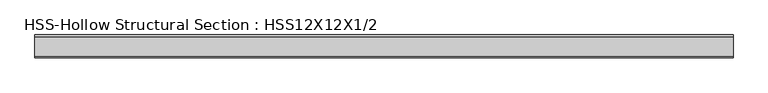
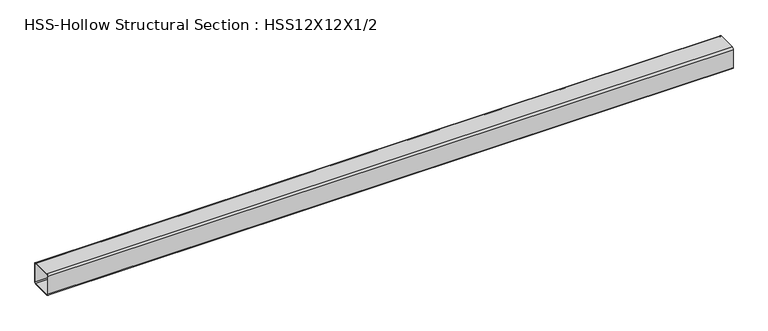
"""IFC4 building model written with IfcOpenShell, lengths in millimetres: beam geometry, HSS-Hollow Structural Section : HSS12X12X1/2."""

import ifcopenshell
import ifcopenshell.guid

model = None  # the IFC model being written
_history = None  # IfcOwnerHistory: only IFC2X3 demands one
_inside = {}  # id of a spatial element -> (the spatial element, [elements in it])
_under = {}  # id of a project, library or spatial element -> (it, [spatial elements below it])
_declared = {}  # id of a project -> (the project, [libraries it declares])
_typed = {}  # id of a type object -> (the type object, [elements of that type])
_made_of = {}  # id of a material, layer set ... -> (it, [elements and type objects made of it])


def new_model(schema):
    """Start an empty IFC model of exactly this schema.

    Asked for "IFC4X3", IfcOpenShell would pick the latest addendum, in which some entities
    have other attributes; the version numbers below select the first issue.
    IFC2X3 requires an IfcOwnerHistory on every rooted entity: one is made here for all.
    """
    global model, _history
    if schema == "IFC4X3":
        model = ifcopenshell.file(schema_version=(4, 3, 0, 0))
    else:
        model = ifcopenshell.file(schema=schema)
    _inside.clear()
    _under.clear()
    _declared.clear()
    _typed.clear()
    _made_of.clear()
    _history = None
    if model.schema == "IFC2X3":
        org = make("IfcOrganization", Name="unknown")
        user = make(
            "IfcPersonAndOrganization",
            ThePerson=make("IfcPerson", FamilyName="unknown"),
            TheOrganization=org,
        )
        app = make(
            "IfcApplication",
            ApplicationDeveloper=org,
            Version="unknown",
            ApplicationFullName="unknown",
            ApplicationIdentifier="unknown",
        )
        _history = make(
            "IfcOwnerHistory",
            OwningUser=user,
            OwningApplication=app,
            ChangeAction="ADDED",
            CreationDate=0,
        )
    return model


def make(cls, **values):
    """One entity of the class cls with the attributes given. An attribute that is None is left unset."""
    return model.create_entity(
        cls, **{name: value for name, value in values.items() if value is not None}
    )


def rooted(cls, **values):
    """An entity with a GlobalId (a new one), such as an element, a storey or a relation."""
    return make(cls, GlobalId=ifcopenshell.guid.new(), OwnerHistory=_history, **values)


def si_unit(unit_type, name, prefix=None):
    """IfcSIUnit, for example si_unit("LENGTHUNIT", "METRE", prefix="MILLI")."""
    return make("IfcSIUnit", UnitType=unit_type, Prefix=prefix, Name=name)


def assignment(units):
    """IfcUnitAssignment: the units of a project."""
    return None if units is None else make("IfcUnitAssignment", Units=units)


def point(xyz):
    """IfcCartesianPoint."""
    return None if xyz is None else make("IfcCartesianPoint", Coordinates=xyz)


def direction(xyz):
    """IfcDirection."""
    return None if xyz is None else make("IfcDirection", DirectionRatios=xyz)


def frame(location, z_axis=None, x_axis=None):
    """IfcAxis2Placement3D, a coordinate frame: its origin and axes. An axis left out is left unset."""
    return make(
        "IfcAxis2Placement3D",
        Location=point(location),
        Axis=direction(z_axis),
        RefDirection=direction(x_axis),
    )


def frame_2d(location, x_axis=None):
    """IfcAxis2Placement2D, a coordinate frame in the plane: its origin and x axis."""
    return make(
        "IfcAxis2Placement2D", Location=point(location), RefDirection=direction(x_axis)
    )


def origin():
    """The frame at (0, 0, 0) with its axes left unset."""
    return frame((0.0, 0.0, 0.0))


def place(relative_to, where):
    """IfcLocalPlacement: puts the frame where relative to a parent placement (None: the world)."""
    return make(
        "IfcLocalPlacement", PlacementRelTo=relative_to, RelativePlacement=where
    )


def context(
    kind, dimensions, precision=None, world=None, true_north=None, identifier=None
):
    """IfcGeometricRepresentationContext, for example the 3D "Model" context."""
    return make(
        "IfcGeometricRepresentationContext",
        ContextIdentifier=identifier,
        ContextType=kind,
        CoordinateSpaceDimension=dimensions,
        Precision=precision,
        WorldCoordinateSystem=world,
        TrueNorth=true_north,
    )


def project(units=None, contexts=None):
    """IfcProject with its units and contexts."""
    return rooted(
        "IfcProject",
        Name="project",
        RepresentationContexts=contexts,
        UnitsInContext=assignment(units),
    )


def spatial(cls, under=None, at=None, **own):
    """A site, building, storey or space (cls), placed at a placement, below another one or the project."""
    s = rooted(cls, ObjectPlacement=at, **own)
    if under is not None:
        _under.setdefault(under.id(), (under, []))[1].append(s)
    return s


def polyline(points):
    """IfcPolyline through the points."""
    return make("IfcPolyline", Points=[point(p) for p in points])


def circle_curve(where, radius):
    """IfcCircle in the frame where."""
    return make("IfcCircle", Position=where, Radius=radius)


def trimmed(basis, trim1, trim2, sense, master):
    """IfcTrimmedCurve: the piece of a basis curve between two trims."""
    return make(
        "IfcTrimmedCurve",
        BasisCurve=basis,
        Trim1=trim1,
        Trim2=trim2,
        SenseAgreement=sense,
        MasterRepresentation=master,
    )


def segment(curve, same_sense, transition):
    """IfcCompositeCurveSegment."""
    return make(
        "IfcCompositeCurveSegment",
        Transition=transition,
        SameSense=same_sense,
        ParentCurve=curve,
    )


def composite_curve(segments, self_intersect=None):
    """IfcCompositeCurve: segments joined end to end."""
    return make("IfcCompositeCurve", Segments=segments, SelfIntersect=self_intersect)


def outline(outer, holes=None, kind="AREA"):
    """IfcArbitraryClosedProfileDef: a profile drawn as a closed curve; with holes, ...WithVoids."""
    if holes is None:
        return make("IfcArbitraryClosedProfileDef", ProfileType=kind, OuterCurve=outer)
    return make(
        "IfcArbitraryProfileDefWithVoids",
        ProfileType=kind,
        OuterCurve=outer,
        InnerCurves=holes,
    )


def extrude(swept, where, along, depth):
    """IfcExtrudedAreaSolid: the profile swept, set in the frame where, extruded along a direction by depth."""
    return make(
        "IfcExtrudedAreaSolid",
        SweptArea=swept,
        Position=where,
        ExtrudedDirection=direction(along),
        Depth=depth,
    )


def shape(context_of_items, identifier, shape_type, items):
    """IfcShapeRepresentation: the items that make up one representation, for example the "Body"."""
    return make(
        "IfcShapeRepresentation",
        ContextOfItems=context_of_items,
        RepresentationIdentifier=identifier,
        RepresentationType=shape_type,
        Items=items,
    )


def source(mapping_origin, context_of_items, identifier, shape_type, items):
    """IfcRepresentationMap: a shape defined once, which mapped items show again and again."""
    return make(
        "IfcRepresentationMap",
        MappingOrigin=mapping_origin,
        MappedRepresentation=shape(context_of_items, identifier, shape_type, items),
    )


def transform(
    local_origin,
    x_axis=None,
    y_axis=None,
    z_axis=None,
    scale=None,
    scale2=None,
    scale3=None,
    uniform=True,
):
    """IfcCartesianTransformationOperator3D, or its non-uniform kind. x_axis, y_axis, z_axis: its Axis1, 2, 3."""
    if uniform:
        return make(
            "IfcCartesianTransformationOperator3D",
            Axis1=direction(x_axis),
            Axis2=direction(y_axis),
            LocalOrigin=point(local_origin),
            Scale=scale,
            Axis3=direction(z_axis),
        )
    return make(
        "IfcCartesianTransformationOperator3DnonUniform",
        Axis1=direction(x_axis),
        Axis2=direction(y_axis),
        LocalOrigin=point(local_origin),
        Scale=scale,
        Axis3=direction(z_axis),
        Scale2=scale2,
        Scale3=scale3,
    )


def mapped(mapping_source, mapping_target):
    """IfcMappedItem: shows the shape of a source again, moved by a transform."""
    return make(
        "IfcMappedItem", MappingSource=mapping_source, MappingTarget=mapping_target
    )


def made_of(thing, what):
    """Note that an element or type object is made of a material, layer set ...; save() writes the relation."""
    if what is not None:
        _made_of.setdefault(what.id(), (what, []))[1].append(thing)
    return thing


def element(
    cls,
    number,
    at=None,
    inside=None,
    cuts=None,
    type_object=None,
    material=None,
    context=None,
    identifier="Body",
    shape_type=None,
    held_by="IfcProductDefinitionShape",
    body=None,
    shapes=None,
    **own,
):
    """One element of the class cls, such as IfcWall. Its Tag is "e" and its number.

    at: its placement. inside: the storey or other place that contains it. cuts: it is an
    opening in that element (IfcRelVoidsElement). A single representation is given by context,
    identifier, shape_type and body (its items); several are given by shapes. held_by: the class
    of the entity that holds the representations. save() writes the other relations.
    """
    e = rooted(cls, Tag="e%d" % number, ObjectPlacement=at, **own)
    if body is not None:
        shapes = [shape(context, identifier, shape_type, body)]
    if shapes is not None:
        e.Representation = make(held_by, Representations=shapes)
    if inside is not None:
        _inside.setdefault(inside.id(), (inside, []))[1].append(e)
    if cuts is not None:
        rooted(
            "IfcRelVoidsElement", RelatingBuildingElement=cuts, RelatedOpeningElement=e
        )
    if type_object is not None:
        _typed.setdefault(type_object.id(), (type_object, []))[1].append(e)
    return made_of(e, material)


def aggregate(whole, parts):
    """IfcRelAggregates: a whole, such as a stair, and the parts it consists of."""
    return rooted("IfcRelAggregates", RelatingObject=whole, RelatedObjects=parts)


def save(model, path):
    """Write the relations noted so far, then the file.

    IfcRelAggregates (storeys below a building ...), IfcRelContainedInSpatialStructure (elements
    in a storey), IfcRelDefinesByType, IfcRelAssociatesMaterial and IfcRelDeclares: one each for
    every whole, place, type object, material and project.
    """
    for whole, parts in _under.values():
        aggregate(whole, parts)
    for where, things in _inside.values():
        rooted(
            "IfcRelContainedInSpatialStructure",
            RelatedElements=things,
            RelatingStructure=where,
        )
    for kind, things in _typed.values():
        rooted("IfcRelDefinesByType", RelatedObjects=things, RelatingType=kind)
    for what, things in _made_of.values():
        rooted("IfcRelAssociatesMaterial", RelatedObjects=things, RelatingMaterial=what)
    for by, libraries in _declared.values():
        rooted("IfcRelDeclares", RelatingContext=by, RelatedDefinitions=libraries)
    model.write(path)


def hss_hollow_structural_section_hss12x12x1_2_75c03b45(model_context):
    return source(origin(), model_context, "Body", "SweptSolid", [
        extrude(outline(composite_curve([segment(polyline([(152.4, 128.778), (152.4, -128.778)]), True, "CONTINUOUS"), segment(trimmed(circle_curve(frame_2d((128.778, -128.778)), 23.622), [point((152.4, -128.778))], [point((128.778, -152.4))], False, "CARTESIAN"), True, "CONTINUOUS"), segment(polyline([(128.778, -152.4), (-128.778, -152.4)]), True, "CONTINUOUS"), segment(trimmed(circle_curve(frame_2d((-128.778, -128.778)), 23.622), [point((-128.778, -152.4))], [point((-152.4, -128.778))], False, "CARTESIAN"), True, "CONTINUOUS"), segment(polyline([(-152.4, -128.778), (-152.4, 128.778)]), True, "CONTINUOUS"), segment(trimmed(circle_curve(frame_2d((-128.778, 128.778)), 23.622), [point((-152.4, 128.778))], [point((-128.778, 152.4))], False, "CARTESIAN"), True, "CONTINUOUS"), segment(polyline([(-128.778, 152.4), (128.778, 152.4)]), True, "CONTINUOUS"), segment(trimmed(circle_curve(frame_2d((128.778, 128.778)), 23.622), [point((128.778, 152.4))], [point((152.4, 128.778))], False, "CARTESIAN"), True, "CONTINUOUS")], self_intersect=False), holes=[composite_curve([segment(trimmed(circle_curve(frame_2d((-128.778, 128.778)), 11.811), [point((-128.778, 140.589))], [point((-140.589, 128.778))], True, "CARTESIAN"), True, "CONTINUOUS"), segment(polyline([(-140.589, 128.778), (-140.589, -128.778)]), True, "CONTINUOUS"), segment(trimmed(circle_curve(frame_2d((-128.778, -128.778)), 11.811), [point((-140.589, -128.778))], [point((-128.778, -140.589))], True, "CARTESIAN"), True, "CONTINUOUS"), segment(polyline([(-128.778, -140.589), (128.778, -140.589)]), True, "CONTINUOUS"), segment(trimmed(circle_curve(frame_2d((128.778, -128.778)), 11.811), [point((128.778, -140.589))], [point((140.589, -128.778))], True, "CARTESIAN"), True, "CONTINUOUS"), segment(polyline([(140.589, -128.778), (140.589, 128.778)]), True, "CONTINUOUS"), segment(trimmed(circle_curve(frame_2d((128.778, 128.778)), 11.811), [point((140.589, 128.778))], [point((128.778, 140.589))], True, "CARTESIAN"), True, "CONTINUOUS"), segment(polyline([(128.778, 140.589), (-128.778, 140.589)]), True, "CONTINUOUS")], self_intersect=False)]), frame((-4705.4254912, 0.0, 0.0), z_axis=(1.0, 0.0, 0.0), x_axis=(0.0, 1.0, 0.0)), (0.0, 0.0, 1.0), 9256.6663725),
    ])


if __name__ == "__main__":
    model = new_model("IFC4")
    model_context = context("Model", 3, world=origin())
    ifc_project = project(units=[si_unit("LENGTHUNIT", "METRE", prefix="MILLI")], contexts=[model_context])
    site = spatial("IfcSite", under=ifc_project)
    building = spatial("IfcBuilding", under=site)
    placement = place(None, origin())
    hss_hollow_structural_section_hss12x12x1_2_shape = hss_hollow_structural_section_hss12x12x1_2_75c03b45(model_context)
    element("IfcBeam", 1, ObjectType="HSS-Hollow Structural Section : HSS12X12X1/2", at=placement, inside=building, context=model_context, shape_type="MappedRepresentation", body=[
        mapped(hss_hollow_structural_section_hss12x12x1_2_shape, transform((0.0, 0.0, 0.0), x_axis=(1.0, 0.0, 0.0), y_axis=(0.0, 1.0, 0.0), z_axis=(0.0, 0.0, 1.0))),
    ])
    save(model, "model.ifc")

# Revit data of these elements
# Type "HSS-Hollow Structural Section : HSS12X12X1/2"
#   Assembly Code = "B10"
#   Shape = "Square"
#   W = 75.9
#   Ht = 304.8 mm
#   Length [instance default] = 1524 mm
#   b = 304.8 mm
#   kr = 23.622 mm
#   t = 11.811 mm
#   A = 0.0134838 m²
#   Structural Material [instance default] = Steel ASTM A500, Grade B, Rectangular and Square
# Element 1 (IfcBeam, "HSS-Hollow Structural Section : HSS12X12X1/2")
#   Structural Material = Aluminum 7175 T73 0 Hot Formed
#   Materials on its faces: "Aluminum 7175 T73 0 Hot Formed"
# Materials
#   "Steel ASTM A500, Grade B, Rectangular and Square": class "Metal", colour RGB 199 199 199, transparency 0, Description = "Carbon steel", Cost = 0
#   "Aluminum 7175 T73 0 Hot Formed": class "Metal", colour RGB 120 120 120, transparency 0, Description = "Physical material.", Cost = 0
